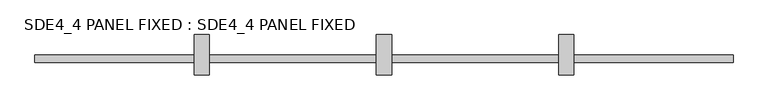
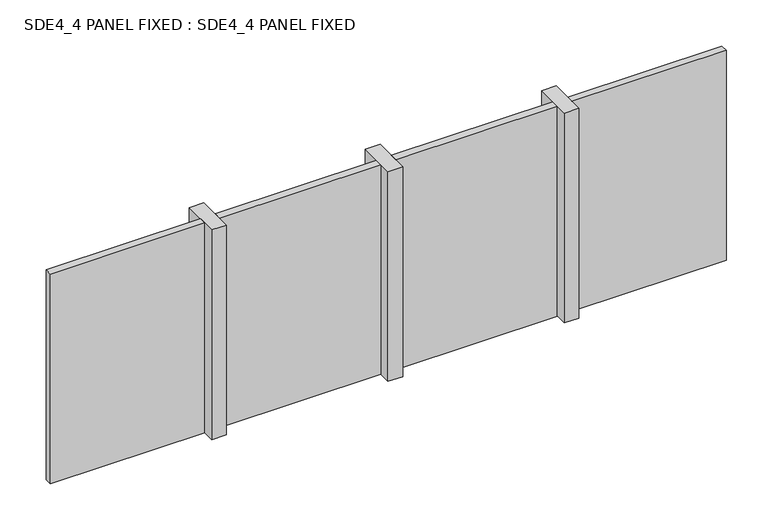
"""IFC4 building model written with IfcOpenShell, lengths in millimetres: plate geometry, SDE4_4 PANEL FIXED : SDE4_4 PANEL FIXED."""

from ifc_helpers import new_model, si_unit, origin, origin_with_axes, place, context, project, spatial, polyline, outline, extrude, source, transform, mapped, element, save


def sde4_4_panel_fixed_sde4_4_panel_fixed_6128f111(model_context):
    return source(origin(), model_context, "Body", "SweptSolid", [
        extrude(outline(polyline([(-1150.0, -132.5), (-1250.0, -132.5), (-1250.0, 132.5), (-1150.0, 132.5), (-1150.0, -132.5)])), origin_with_axes(), (0.0, 0.0, 1.0), 1510.0),
        extrude(outline(polyline([(50.0, -132.5), (-50.0, -132.5), (-50.0, 132.5), (50.0, 132.5), (50.0, -132.5)])), origin_with_axes(), (0.0, 0.0, 1.0), 1510.0),
        extrude(outline(polyline([(1250.0, -132.5), (1150.0, -132.5), (1150.0, 132.5), (1250.0, 132.5), (1250.0, -132.5)])), origin_with_axes(), (0.0, 0.0, 1.0), 1510.0),
        extrude(outline(polyline([(2299.0, -50.0), (1250.0, -50.0), (1250.0, 0.0), (2299.0, 0.0), (2299.0, -50.0)])), origin_with_axes(), (0.0, 0.0, 1.0), 1510.0),
        extrude(outline(polyline([(1150.0, -50.0), (50.0, -50.0), (50.0, 0.0), (1150.0, 0.0), (1150.0, -50.0)])), origin_with_axes(), (0.0, 0.0, 1.0), 1510.0),
        extrude(outline(polyline([(-50.0, -50.0), (-1150.0, -50.0), (-1150.0, 0.0), (-50.0, 0.0), (-50.0, -50.0)])), origin_with_axes(), (0.0, 0.0, 1.0), 1510.0),
        extrude(outline(polyline([(-1250.0, -50.0), (-2300.0, -50.0), (-2300.0, 0.0), (-1250.0, 0.0), (-1250.0, -50.0)])), origin_with_axes(), (0.0, 0.0, 1.0), 1510.0),
    ])


if __name__ == "__main__":
    model = new_model("IFC4")
    model_context = context("Model", 3, world=origin())
    ifc_project = project(units=[si_unit("LENGTHUNIT", "METRE", prefix="MILLI")], contexts=[model_context])
    site = spatial("IfcSite", under=ifc_project)
    building = spatial("IfcBuilding", under=site)
    placement = place(None, origin())
    sde4_4_panel_fixed_sde4_4_panel_fixed_shape = sde4_4_panel_fixed_sde4_4_panel_fixed_6128f111(model_context)
    element("IfcPlate", 1, ObjectType="SDE4_4 PANEL FIXED : SDE4_4 PANEL FIXED", at=placement, inside=building, context=model_context, shape_type="MappedRepresentation", body=[
        mapped(sde4_4_panel_fixed_sde4_4_panel_fixed_shape, transform((0.0, 0.0, 0.0), x_axis=(1.0, 0.0, 0.0), y_axis=(0.0, 1.0, 0.0), z_axis=(0.0, 0.0, 1.0))),
    ])
    save(model, "model.ifc")

# Revit data of these elements
# Type "SDE4_4 PANEL FIXED : SDE4_4 PANEL FIXED"
#   Type Mark = "CW-GLASS"
#   Analytic Construction = "<None>"
#   Glass = Glass
#   Frame = Aluminium
# Element 1 (IfcPlate, "SDE4_4 PANEL FIXED : SDE4_4 PANEL FIXED")
#   Materials on its faces: "Glass", "Aluminium"
# Materials
#   "Glass": class "Glass", colour RGB 0 128 192, transparency 0.9, Keynote = "L40", Cost = 0
#   "Aluminium": class "Unassigned", colour RGB 247 247 247, transparency 0, Cost = 0
